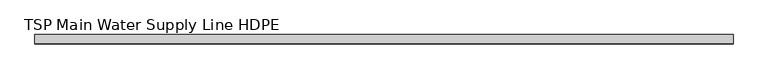
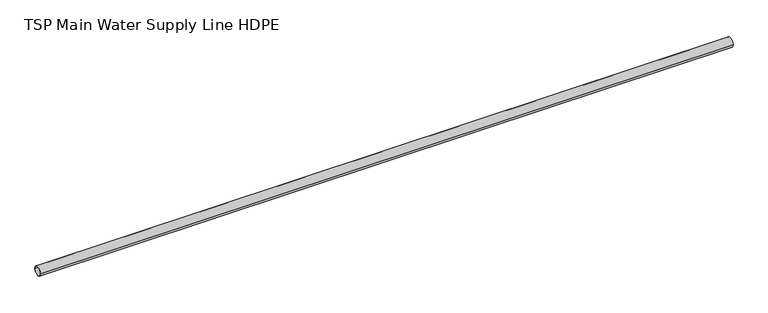
"""IFC4 building model written with IfcOpenShell, lengths in millimetres: flow terminal geometry, TSP Main Water Supply Line HDPE : HDPE Fresh Water Supply."""

import ifcopenshell
import ifcopenshell.guid

model = None  # the IFC model being written
_history = None  # IfcOwnerHistory: only IFC2X3 demands one
_inside = {}  # id of a spatial element -> (the spatial element, [elements in it])
_under = {}  # id of a project, library or spatial element -> (it, [spatial elements below it])
_declared = {}  # id of a project -> (the project, [libraries it declares])
_typed = {}  # id of a type object -> (the type object, [elements of that type])
_made_of = {}  # id of a material, layer set ... -> (it, [elements and type objects made of it])


def new_model(schema):
    """Start an empty IFC model of exactly this schema.

    Asked for "IFC4X3", IfcOpenShell would pick the latest addendum, in which some entities
    have other attributes; the version numbers below select the first issue.
    IFC2X3 requires an IfcOwnerHistory on every rooted entity: one is made here for all.
    """
    global model, _history
    if schema == "IFC4X3":
        model = ifcopenshell.file(schema_version=(4, 3, 0, 0))
    else:
        model = ifcopenshell.file(schema=schema)
    _inside.clear()
    _under.clear()
    _declared.clear()
    _typed.clear()
    _made_of.clear()
    _history = None
    if model.schema == "IFC2X3":
        org = make("IfcOrganization", Name="unknown")
        user = make(
            "IfcPersonAndOrganization",
            ThePerson=make("IfcPerson", FamilyName="unknown"),
            TheOrganization=org,
        )
        app = make(
            "IfcApplication",
            ApplicationDeveloper=org,
            Version="unknown",
            ApplicationFullName="unknown",
            ApplicationIdentifier="unknown",
        )
        _history = make(
            "IfcOwnerHistory",
            OwningUser=user,
            OwningApplication=app,
            ChangeAction="ADDED",
            CreationDate=0,
        )
    return model


def make(cls, **values):
    """One entity of the class cls with the attributes given. An attribute that is None is left unset."""
    return model.create_entity(
        cls, **{name: value for name, value in values.items() if value is not None}
    )


def rooted(cls, **values):
    """An entity with a GlobalId (a new one), such as an element, a storey or a relation."""
    return make(cls, GlobalId=ifcopenshell.guid.new(), OwnerHistory=_history, **values)


def si_unit(unit_type, name, prefix=None):
    """IfcSIUnit, for example si_unit("LENGTHUNIT", "METRE", prefix="MILLI")."""
    return make("IfcSIUnit", UnitType=unit_type, Prefix=prefix, Name=name)


def assignment(units):
    """IfcUnitAssignment: the units of a project."""
    return None if units is None else make("IfcUnitAssignment", Units=units)


def point(xyz):
    """IfcCartesianPoint."""
    return None if xyz is None else make("IfcCartesianPoint", Coordinates=xyz)


def direction(xyz):
    """IfcDirection."""
    return None if xyz is None else make("IfcDirection", DirectionRatios=xyz)


def frame(location, z_axis=None, x_axis=None):
    """IfcAxis2Placement3D, a coordinate frame: its origin and axes. An axis left out is left unset."""
    return make(
        "IfcAxis2Placement3D",
        Location=point(location),
        Axis=direction(z_axis),
        RefDirection=direction(x_axis),
    )


def frame_2d(location, x_axis=None):
    """IfcAxis2Placement2D, a coordinate frame in the plane: its origin and x axis."""
    return make(
        "IfcAxis2Placement2D", Location=point(location), RefDirection=direction(x_axis)
    )


def origin():
    """The frame at (0, 0, 0) with its axes left unset."""
    return frame((0.0, 0.0, 0.0))


def origin_2d():
    """The frame at (0, 0) in the plane with its x axis left unset."""
    return frame_2d((0.0, 0.0))


def place(relative_to, where):
    """IfcLocalPlacement: puts the frame where relative to a parent placement (None: the world)."""
    return make(
        "IfcLocalPlacement", PlacementRelTo=relative_to, RelativePlacement=where
    )


def context(
    kind, dimensions, precision=None, world=None, true_north=None, identifier=None
):
    """IfcGeometricRepresentationContext, for example the 3D "Model" context."""
    return make(
        "IfcGeometricRepresentationContext",
        ContextIdentifier=identifier,
        ContextType=kind,
        CoordinateSpaceDimension=dimensions,
        Precision=precision,
        WorldCoordinateSystem=world,
        TrueNorth=true_north,
    )


def project(units=None, contexts=None):
    """IfcProject with its units and contexts."""
    return rooted(
        "IfcProject",
        Name="project",
        RepresentationContexts=contexts,
        UnitsInContext=assignment(units),
    )


def spatial(cls, under=None, at=None, **own):
    """A site, building, storey or space (cls), placed at a placement, below another one or the project."""
    s = rooted(cls, ObjectPlacement=at, **own)
    if under is not None:
        _under.setdefault(under.id(), (under, []))[1].append(s)
    return s


def circle_curve(where, radius):
    """IfcCircle in the frame where."""
    return make("IfcCircle", Position=where, Radius=radius)


def trimmed(basis, trim1, trim2, sense, master):
    """IfcTrimmedCurve: the piece of a basis curve between two trims."""
    return make(
        "IfcTrimmedCurve",
        BasisCurve=basis,
        Trim1=trim1,
        Trim2=trim2,
        SenseAgreement=sense,
        MasterRepresentation=master,
    )


def segment(curve, same_sense, transition):
    """IfcCompositeCurveSegment."""
    return make(
        "IfcCompositeCurveSegment",
        Transition=transition,
        SameSense=same_sense,
        ParentCurve=curve,
    )


def composite_curve(segments, self_intersect=None):
    """IfcCompositeCurve: segments joined end to end."""
    return make("IfcCompositeCurve", Segments=segments, SelfIntersect=self_intersect)


def outline(outer, holes=None, kind="AREA"):
    """IfcArbitraryClosedProfileDef: a profile drawn as a closed curve; with holes, ...WithVoids."""
    if holes is None:
        return make("IfcArbitraryClosedProfileDef", ProfileType=kind, OuterCurve=outer)
    return make(
        "IfcArbitraryProfileDefWithVoids",
        ProfileType=kind,
        OuterCurve=outer,
        InnerCurves=holes,
    )


def extrude(swept, where, along, depth):
    """IfcExtrudedAreaSolid: the profile swept, set in the frame where, extruded along a direction by depth."""
    return make(
        "IfcExtrudedAreaSolid",
        SweptArea=swept,
        Position=where,
        ExtrudedDirection=direction(along),
        Depth=depth,
    )


def shape(context_of_items, identifier, shape_type, items):
    """IfcShapeRepresentation: the items that make up one representation, for example the "Body"."""
    return make(
        "IfcShapeRepresentation",
        ContextOfItems=context_of_items,
        RepresentationIdentifier=identifier,
        RepresentationType=shape_type,
        Items=items,
    )


def source(mapping_origin, context_of_items, identifier, shape_type, items):
    """IfcRepresentationMap: a shape defined once, which mapped items show again and again."""
    return make(
        "IfcRepresentationMap",
        MappingOrigin=mapping_origin,
        MappedRepresentation=shape(context_of_items, identifier, shape_type, items),
    )


def transform(
    local_origin,
    x_axis=None,
    y_axis=None,
    z_axis=None,
    scale=None,
    scale2=None,
    scale3=None,
    uniform=True,
):
    """IfcCartesianTransformationOperator3D, or its non-uniform kind. x_axis, y_axis, z_axis: its Axis1, 2, 3."""
    if uniform:
        return make(
            "IfcCartesianTransformationOperator3D",
            Axis1=direction(x_axis),
            Axis2=direction(y_axis),
            LocalOrigin=point(local_origin),
            Scale=scale,
            Axis3=direction(z_axis),
        )
    return make(
        "IfcCartesianTransformationOperator3DnonUniform",
        Axis1=direction(x_axis),
        Axis2=direction(y_axis),
        LocalOrigin=point(local_origin),
        Scale=scale,
        Axis3=direction(z_axis),
        Scale2=scale2,
        Scale3=scale3,
    )


def mapped(mapping_source, mapping_target):
    """IfcMappedItem: shows the shape of a source again, moved by a transform."""
    return make(
        "IfcMappedItem", MappingSource=mapping_source, MappingTarget=mapping_target
    )


def made_of(thing, what):
    """Note that an element or type object is made of a material, layer set ...; save() writes the relation."""
    if what is not None:
        _made_of.setdefault(what.id(), (what, []))[1].append(thing)
    return thing


def element(
    cls,
    number,
    at=None,
    inside=None,
    cuts=None,
    type_object=None,
    material=None,
    context=None,
    identifier="Body",
    shape_type=None,
    held_by="IfcProductDefinitionShape",
    body=None,
    shapes=None,
    **own,
):
    """One element of the class cls, such as IfcWall. Its Tag is "e" and its number.

    at: its placement. inside: the storey or other place that contains it. cuts: it is an
    opening in that element (IfcRelVoidsElement). A single representation is given by context,
    identifier, shape_type and body (its items); several are given by shapes. held_by: the class
    of the entity that holds the representations. save() writes the other relations.
    """
    e = rooted(cls, Tag="e%d" % number, ObjectPlacement=at, **own)
    if body is not None:
        shapes = [shape(context, identifier, shape_type, body)]
    if shapes is not None:
        e.Representation = make(held_by, Representations=shapes)
    if inside is not None:
        _inside.setdefault(inside.id(), (inside, []))[1].append(e)
    if cuts is not None:
        rooted(
            "IfcRelVoidsElement", RelatingBuildingElement=cuts, RelatedOpeningElement=e
        )
    if type_object is not None:
        _typed.setdefault(type_object.id(), (type_object, []))[1].append(e)
    return made_of(e, material)


def aggregate(whole, parts):
    """IfcRelAggregates: a whole, such as a stair, and the parts it consists of."""
    return rooted("IfcRelAggregates", RelatingObject=whole, RelatedObjects=parts)


def save(model, path):
    """Write the relations noted so far, then the file.

    IfcRelAggregates (storeys below a building ...), IfcRelContainedInSpatialStructure (elements
    in a storey), IfcRelDefinesByType, IfcRelAssociatesMaterial and IfcRelDeclares: one each for
    every whole, place, type object, material and project.
    """
    for whole, parts in _under.values():
        aggregate(whole, parts)
    for where, things in _inside.values():
        rooted(
            "IfcRelContainedInSpatialStructure",
            RelatedElements=things,
            RelatingStructure=where,
        )
    for kind, things in _typed.values():
        rooted("IfcRelDefinesByType", RelatedObjects=things, RelatingType=kind)
    for what, things in _made_of.values():
        rooted("IfcRelAssociatesMaterial", RelatedObjects=things, RelatingMaterial=what)
    for by, libraries in _declared.values():
        rooted("IfcRelDeclares", RelatingContext=by, RelatedDefinitions=libraries)
    model.write(path)


def tsp_main_water_supply_line_hdpe_ea8c98fe(model_context):
    return source(origin(), model_context, "Body", "SweptSolid", [
        extrude(outline(composite_curve([segment(trimmed(circle_curve(origin_2d(), 16.0), [point((-16.0, 0.0))], [point((16.0, 0.0))], False, "CARTESIAN"), True, "CONTINUOUS"), segment(trimmed(circle_curve(origin_2d(), 16.0), [point((16.0, 0.0))], [point((-16.0, 0.0))], False, "CARTESIAN"), True, "CONTINUOUS")], self_intersect=False), holes=[composite_curve([segment(trimmed(circle_curve(origin_2d(), 15.0), [point((-15.0, 0.0))], [point((15.0, 0.0))], True, "CARTESIAN"), True, "CONTINUOUS"), segment(trimmed(circle_curve(origin_2d(), 15.0), [point((15.0, 0.0))], [point((-15.0, 0.0))], True, "CARTESIAN"), True, "CONTINUOUS")], self_intersect=False)]), frame((0.0, 0.0, 0.0), z_axis=(1.0, 0.0, 0.0), x_axis=(0.0, 1.0, 0.0)), (0.0, 0.0, 1.0), 2377.9927822),
    ])


if __name__ == "__main__":
    model = new_model("IFC4")
    model_context = context("Model", 3, world=origin())
    ifc_project = project(units=[si_unit("LENGTHUNIT", "METRE", prefix="MILLI")], contexts=[model_context])
    site = spatial("IfcSite", under=ifc_project)
    building = spatial("IfcBuilding", under=site)
    placement = place(None, origin())
    tsp_main_water_supply_line_hdpe_shape = tsp_main_water_supply_line_hdpe_ea8c98fe(model_context)
    element("IfcFlowTerminal", 1, ObjectType="TSP Main Water Supply Line HDPE : HDPE Fresh Water Supply", at=placement, inside=building, context=model_context, shape_type="MappedRepresentation", body=[
        mapped(tsp_main_water_supply_line_hdpe_shape, transform((0.0, 0.0, 0.0), x_axis=(1.0, 0.0, 0.0), y_axis=(0.0, 1.0, 0.0), z_axis=(0.0, 0.0, 1.0))),
    ])
    save(model, "model.ifc")

# Revit data of these elements
# Type "TSP Main Water Supply Line HDPE : HDPE Fresh Water Supply"
#   Model = "TSP_110SFWSP"
#   Pipe length [instance default] = 1200 mm
#   Pipe dia = 30 mm
#   built-in parameter 1001306 [instance default] = 3.93701 (stored number, unit not read)
#   Default Elevation = 0
# Element 1 (IfcFlowTerminal, "TSP Main Water Supply Line HDPE : HDPE Fresh Water Supply")
#   Pipe length = 2377.993 mm
#   built-in parameter 1001306 = 7.80181 (stored number, unit not read)
#   Materials on its faces: "Aluminum, Anodized Blue"
# Materials
#   "Aluminum, Anodized Blue": class "Metal", colour RGB 120 120 120, transparency 0, Description = "Anodized aluminum, blue", Cost = 0
